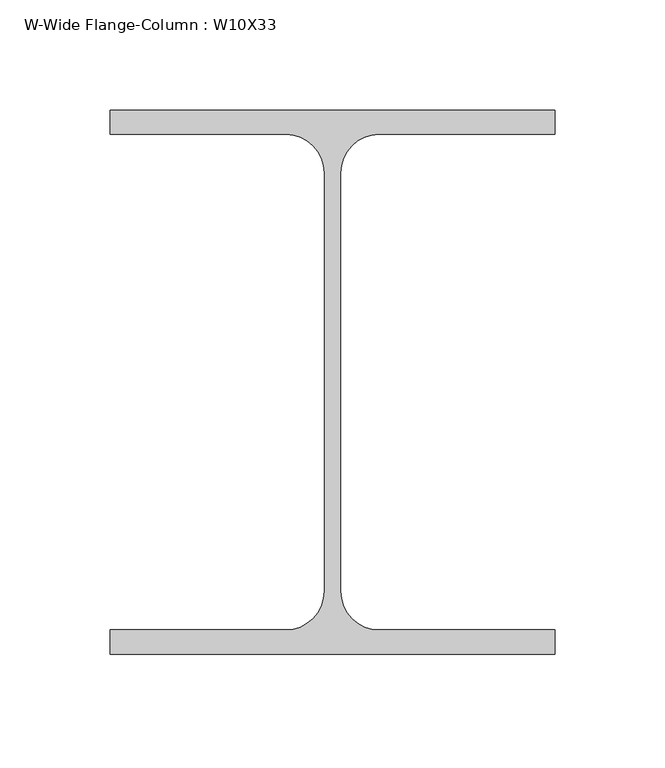
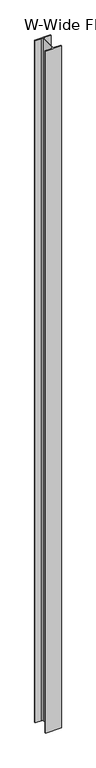
"""IFC4 building model written with IfcOpenShell, lengths in millimetres: column geometry, W-Wide Flange-Column : W10X33."""

import ifcopenshell
import ifcopenshell.guid

model = None  # the IFC model being written
_history = None  # IfcOwnerHistory: only IFC2X3 demands one
_inside = {}  # id of a spatial element -> (the spatial element, [elements in it])
_under = {}  # id of a project, library or spatial element -> (it, [spatial elements below it])
_declared = {}  # id of a project -> (the project, [libraries it declares])
_typed = {}  # id of a type object -> (the type object, [elements of that type])
_made_of = {}  # id of a material, layer set ... -> (it, [elements and type objects made of it])


def new_model(schema):
    """Start an empty IFC model of exactly this schema.

    Asked for "IFC4X3", IfcOpenShell would pick the latest addendum, in which some entities
    have other attributes; the version numbers below select the first issue.
    IFC2X3 requires an IfcOwnerHistory on every rooted entity: one is made here for all.
    """
    global model, _history
    if schema == "IFC4X3":
        model = ifcopenshell.file(schema_version=(4, 3, 0, 0))
    else:
        model = ifcopenshell.file(schema=schema)
    _inside.clear()
    _under.clear()
    _declared.clear()
    _typed.clear()
    _made_of.clear()
    _history = None
    if model.schema == "IFC2X3":
        org = make("IfcOrganization", Name="unknown")
        user = make(
            "IfcPersonAndOrganization",
            ThePerson=make("IfcPerson", FamilyName="unknown"),
            TheOrganization=org,
        )
        app = make(
            "IfcApplication",
            ApplicationDeveloper=org,
            Version="unknown",
            ApplicationFullName="unknown",
            ApplicationIdentifier="unknown",
        )
        _history = make(
            "IfcOwnerHistory",
            OwningUser=user,
            OwningApplication=app,
            ChangeAction="ADDED",
            CreationDate=0,
        )
    return model


def make(cls, **values):
    """One entity of the class cls with the attributes given. An attribute that is None is left unset."""
    return model.create_entity(
        cls, **{name: value for name, value in values.items() if value is not None}
    )


def rooted(cls, **values):
    """An entity with a GlobalId (a new one), such as an element, a storey or a relation."""
    return make(cls, GlobalId=ifcopenshell.guid.new(), OwnerHistory=_history, **values)


def si_unit(unit_type, name, prefix=None):
    """IfcSIUnit, for example si_unit("LENGTHUNIT", "METRE", prefix="MILLI")."""
    return make("IfcSIUnit", UnitType=unit_type, Prefix=prefix, Name=name)


def assignment(units):
    """IfcUnitAssignment: the units of a project."""
    return None if units is None else make("IfcUnitAssignment", Units=units)


def point(xyz):
    """IfcCartesianPoint."""
    return None if xyz is None else make("IfcCartesianPoint", Coordinates=xyz)


def direction(xyz):
    """IfcDirection."""
    return None if xyz is None else make("IfcDirection", DirectionRatios=xyz)


def frame(location, z_axis=None, x_axis=None):
    """IfcAxis2Placement3D, a coordinate frame: its origin and axes. An axis left out is left unset."""
    return make(
        "IfcAxis2Placement3D",
        Location=point(location),
        Axis=direction(z_axis),
        RefDirection=direction(x_axis),
    )


def frame_2d(location, x_axis=None):
    """IfcAxis2Placement2D, a coordinate frame in the plane: its origin and x axis."""
    return make(
        "IfcAxis2Placement2D", Location=point(location), RefDirection=direction(x_axis)
    )


def origin():
    """The frame at (0, 0, 0) with its axes left unset."""
    return frame((0.0, 0.0, 0.0))


def place(relative_to, where):
    """IfcLocalPlacement: puts the frame where relative to a parent placement (None: the world)."""
    return make(
        "IfcLocalPlacement", PlacementRelTo=relative_to, RelativePlacement=where
    )


def context(
    kind, dimensions, precision=None, world=None, true_north=None, identifier=None
):
    """IfcGeometricRepresentationContext, for example the 3D "Model" context."""
    return make(
        "IfcGeometricRepresentationContext",
        ContextIdentifier=identifier,
        ContextType=kind,
        CoordinateSpaceDimension=dimensions,
        Precision=precision,
        WorldCoordinateSystem=world,
        TrueNorth=true_north,
    )


def project(units=None, contexts=None):
    """IfcProject with its units and contexts."""
    return rooted(
        "IfcProject",
        Name="project",
        RepresentationContexts=contexts,
        UnitsInContext=assignment(units),
    )


def spatial(cls, under=None, at=None, **own):
    """A site, building, storey or space (cls), placed at a placement, below another one or the project."""
    s = rooted(cls, ObjectPlacement=at, **own)
    if under is not None:
        _under.setdefault(under.id(), (under, []))[1].append(s)
    return s


def polyline(points):
    """IfcPolyline through the points."""
    return make("IfcPolyline", Points=[point(p) for p in points])


def circle_curve(where, radius):
    """IfcCircle in the frame where."""
    return make("IfcCircle", Position=where, Radius=radius)


def trimmed(basis, trim1, trim2, sense, master):
    """IfcTrimmedCurve: the piece of a basis curve between two trims."""
    return make(
        "IfcTrimmedCurve",
        BasisCurve=basis,
        Trim1=trim1,
        Trim2=trim2,
        SenseAgreement=sense,
        MasterRepresentation=master,
    )


def segment(curve, same_sense, transition):
    """IfcCompositeCurveSegment."""
    return make(
        "IfcCompositeCurveSegment",
        Transition=transition,
        SameSense=same_sense,
        ParentCurve=curve,
    )


def composite_curve(segments, self_intersect=None):
    """IfcCompositeCurve: segments joined end to end."""
    return make("IfcCompositeCurve", Segments=segments, SelfIntersect=self_intersect)


def outline(outer, holes=None, kind="AREA"):
    """IfcArbitraryClosedProfileDef: a profile drawn as a closed curve; with holes, ...WithVoids."""
    if holes is None:
        return make("IfcArbitraryClosedProfileDef", ProfileType=kind, OuterCurve=outer)
    return make(
        "IfcArbitraryProfileDefWithVoids",
        ProfileType=kind,
        OuterCurve=outer,
        InnerCurves=holes,
    )


def extrude(swept, where, along, depth):
    """IfcExtrudedAreaSolid: the profile swept, set in the frame where, extruded along a direction by depth."""
    return make(
        "IfcExtrudedAreaSolid",
        SweptArea=swept,
        Position=where,
        ExtrudedDirection=direction(along),
        Depth=depth,
    )


def shape(context_of_items, identifier, shape_type, items):
    """IfcShapeRepresentation: the items that make up one representation, for example the "Body"."""
    return make(
        "IfcShapeRepresentation",
        ContextOfItems=context_of_items,
        RepresentationIdentifier=identifier,
        RepresentationType=shape_type,
        Items=items,
    )


def source(mapping_origin, context_of_items, identifier, shape_type, items):
    """IfcRepresentationMap: a shape defined once, which mapped items show again and again."""
    return make(
        "IfcRepresentationMap",
        MappingOrigin=mapping_origin,
        MappedRepresentation=shape(context_of_items, identifier, shape_type, items),
    )


def transform(
    local_origin,
    x_axis=None,
    y_axis=None,
    z_axis=None,
    scale=None,
    scale2=None,
    scale3=None,
    uniform=True,
):
    """IfcCartesianTransformationOperator3D, or its non-uniform kind. x_axis, y_axis, z_axis: its Axis1, 2, 3."""
    if uniform:
        return make(
            "IfcCartesianTransformationOperator3D",
            Axis1=direction(x_axis),
            Axis2=direction(y_axis),
            LocalOrigin=point(local_origin),
            Scale=scale,
            Axis3=direction(z_axis),
        )
    return make(
        "IfcCartesianTransformationOperator3DnonUniform",
        Axis1=direction(x_axis),
        Axis2=direction(y_axis),
        LocalOrigin=point(local_origin),
        Scale=scale,
        Axis3=direction(z_axis),
        Scale2=scale2,
        Scale3=scale3,
    )


def mapped(mapping_source, mapping_target):
    """IfcMappedItem: shows the shape of a source again, moved by a transform."""
    return make(
        "IfcMappedItem", MappingSource=mapping_source, MappingTarget=mapping_target
    )


def made_of(thing, what):
    """Note that an element or type object is made of a material, layer set ...; save() writes the relation."""
    if what is not None:
        _made_of.setdefault(what.id(), (what, []))[1].append(thing)
    return thing


def element(
    cls,
    number,
    at=None,
    inside=None,
    cuts=None,
    type_object=None,
    material=None,
    context=None,
    identifier="Body",
    shape_type=None,
    held_by="IfcProductDefinitionShape",
    body=None,
    shapes=None,
    **own,
):
    """One element of the class cls, such as IfcWall. Its Tag is "e" and its number.

    at: its placement. inside: the storey or other place that contains it. cuts: it is an
    opening in that element (IfcRelVoidsElement). A single representation is given by context,
    identifier, shape_type and body (its items); several are given by shapes. held_by: the class
    of the entity that holds the representations. save() writes the other relations.
    """
    e = rooted(cls, Tag="e%d" % number, ObjectPlacement=at, **own)
    if body is not None:
        shapes = [shape(context, identifier, shape_type, body)]
    if shapes is not None:
        e.Representation = make(held_by, Representations=shapes)
    if inside is not None:
        _inside.setdefault(inside.id(), (inside, []))[1].append(e)
    if cuts is not None:
        rooted(
            "IfcRelVoidsElement", RelatingBuildingElement=cuts, RelatedOpeningElement=e
        )
    if type_object is not None:
        _typed.setdefault(type_object.id(), (type_object, []))[1].append(e)
    return made_of(e, material)


def aggregate(whole, parts):
    """IfcRelAggregates: a whole, such as a stair, and the parts it consists of."""
    return rooted("IfcRelAggregates", RelatingObject=whole, RelatedObjects=parts)


def save(model, path):
    """Write the relations noted so far, then the file.

    IfcRelAggregates (storeys below a building ...), IfcRelContainedInSpatialStructure (elements
    in a storey), IfcRelDefinesByType, IfcRelAssociatesMaterial and IfcRelDeclares: one each for
    every whole, place, type object, material and project.
    """
    for whole, parts in _under.values():
        aggregate(whole, parts)
    for where, things in _inside.values():
        rooted(
            "IfcRelContainedInSpatialStructure",
            RelatedElements=things,
            RelatingStructure=where,
        )
    for kind, things in _typed.values():
        rooted("IfcRelDefinesByType", RelatedObjects=things, RelatingType=kind)
    for what, things in _made_of.values():
        rooted("IfcRelAssociatesMaterial", RelatedObjects=things, RelatingMaterial=what)
    for by, libraries in _declared.values():
        rooted("IfcRelDeclares", RelatingContext=by, RelatedDefinitions=libraries)
    model.write(path)


def w_wide_flange_column_w10x33_efc84e3e(model_context):
    return source(origin(), model_context, "Body", "SweptSolid", [
        extrude(outline(composite_curve([segment(polyline([(101.092, 123.571), (101.092, 112.522), (21.209, 112.522)]), True, "CONTINUOUS"), segment(trimmed(circle_curve(frame_2d((21.209, 94.996)), 17.526), [point((21.209, 112.522))], [point((3.683, 94.996))], True, "CARTESIAN"), True, "CONTINUOUS"), segment(polyline([(3.683, 94.996), (3.683, -94.996)]), True, "CONTINUOUS"), segment(trimmed(circle_curve(frame_2d((21.209, -94.996)), 17.526), [point((3.683, -94.996))], [point((21.209, -112.522))], True, "CARTESIAN"), True, "CONTINUOUS"), segment(polyline([(21.209, -112.522), (101.092, -112.522), (101.092, -123.571), (-101.092, -123.571), (-101.092, -112.522), (-21.209, -112.522)]), True, "CONTINUOUS"), segment(trimmed(circle_curve(frame_2d((-21.209, -94.996)), 17.526), [point((-21.209, -112.522))], [point((-3.683, -94.996))], True, "CARTESIAN"), True, "CONTINUOUS"), segment(polyline([(-3.683, -94.996), (-3.683, 94.996)]), True, "CONTINUOUS"), segment(trimmed(circle_curve(frame_2d((-21.209, 94.996)), 17.526), [point((-3.683, 94.996))], [point((-21.209, 112.522))], True, "CARTESIAN"), True, "CONTINUOUS"), segment(polyline([(-21.209, 112.522), (-101.092, 112.522), (-101.092, 123.571), (101.092, 123.571)]), True, "CONTINUOUS")], self_intersect=False)), frame((0.0, 0.0, 12566.65), z_axis=(0.0, 0.0, 1.0), x_axis=(1.0, 0.0, 0.0)), (0.0, 0.0, 1.0), 9328.15),
    ])


if __name__ == "__main__":
    model = new_model("IFC4")
    model_context = context("Model", 3, world=origin())
    ifc_project = project(units=[si_unit("LENGTHUNIT", "METRE", prefix="MILLI")], contexts=[model_context])
    site = spatial("IfcSite", under=ifc_project)
    building = spatial("IfcBuilding", under=site)
    placement = place(None, origin())
    w_wide_flange_column_w10x33_shape = w_wide_flange_column_w10x33_efc84e3e(model_context)
    element("IfcColumn", 1, ObjectType="W-Wide Flange-Column : W10X33", at=placement, inside=building, context=model_context, shape_type="MappedRepresentation", body=[
        mapped(w_wide_flange_column_w10x33_shape, transform((0.0, 0.0, 0.0), x_axis=(1.0, 0.0, 0.0), y_axis=(0.0, 1.0, 0.0), z_axis=(0.0, 0.0, 1.0))),
    ])
    save(model, "model.ifc")

# Revit data of these elements
# Type "W-Wide Flange-Column : W10X33"
#   Assembly Code = "B10"
#   W = 33
#   bf = 0' - 7.96"
#   d = 0' - 9.73"
#   k = 0' - 1 1/8"
#   kr = 0' - 0.69"
#   tf = 0' - 0.435"
#   tw = 0' - 0.29"
#   A = 0.0674306 SF
#   Structural Material [instance default] = Steel ASTM A992
# Element 1 (IfcColumn, "W-Wide Flange-Column : W10X33")
#   Materials on its faces: "Steel ASTM A992"
# Materials
#   "Steel ASTM A992": class "Metal", colour RGB 199 199 199, transparency 0, Description = "Structural steel 50ksi", Cost = 0
